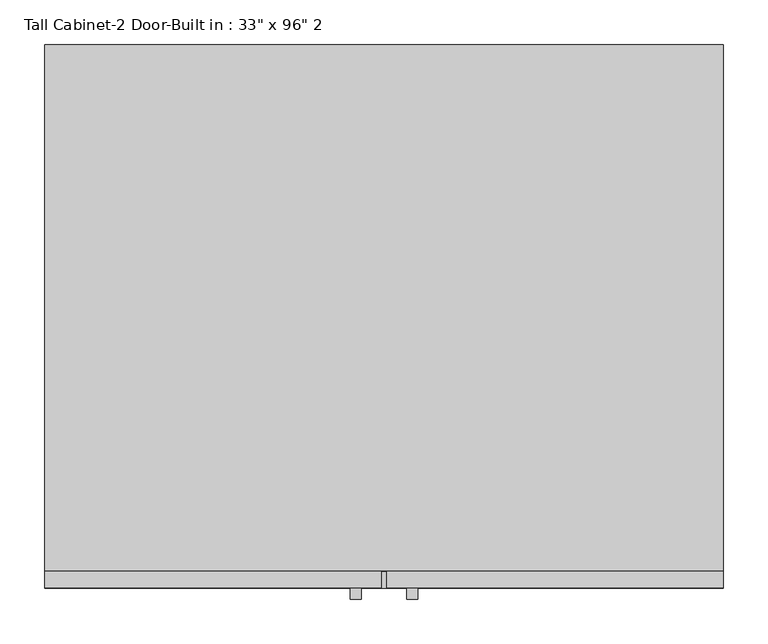
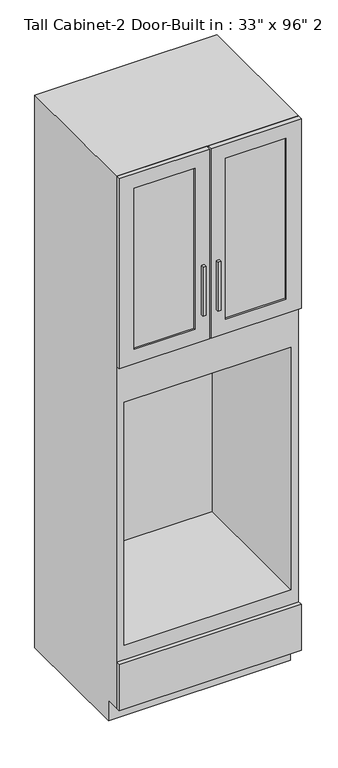
"""IFC4 building model written with IfcOpenShell, lengths in millimetres: furniture geometry."""

from ifc_helpers import new_model, si_unit, frame, origin, place, context, project, spatial, polyline, outline, extrude, faceted_brep, source, transform, mapped, element, save


def furniture_01bc0a7d(model_context):
    return source(origin(), model_context, "Body", "SolidModel", [
        faceted_brep([(399.7377049, -590.55, 90.4875), (399.7377049, -590.55, 2439.9875), (-362.2622951, -590.55, 2439.9875), (-362.2622951, -590.55, 90.4875), (-343.2122951, -590.55, 2420.9375), (380.6877049, -590.55, 2420.9375), (380.6877049, -590.55, 1601.7875), (-343.2122951, -590.55, 1601.7875), (367.9877049, -590.55, 357.1875), (-330.5122951, -590.55, 357.1875), (-330.5122951, -590.55, 1430.3375), (367.9877049, -590.55, 1430.3375), (-362.2622951, 0.0, 2439.9875), (399.7377049, 0.0, 2439.9875), (399.7377049, 0.0, 0.0), (-362.2622951, 0.0, 0.0), (399.7377049, -533.4, 90.4875), (399.7377049, -533.4, 0.0), (-362.2622951, -533.4, 0.0), (-362.2622951, -533.4, 90.4875), (380.6877049, -19.05, 2420.9375), (380.6877049, -19.05, 1601.7875), (-343.2122951, -19.05, 1601.7875), (-343.2122951, -19.05, 2420.9375), (367.9877049, -19.05, 357.1875), (-330.5122951, -19.05, 357.1875), (-330.5122951, -19.05, 1430.3375), (367.9877049, -19.05, 1430.3375)], [[[0, 1, 2, 3], [4, 5, 6, 7], [8, 9, 10, 11]], [[12, 13, 14, 15]], [[1, 0, 16, 17, 14, 13]], [[2, 1, 13, 12]], [[3, 2, 12, 15, 18, 19]], [[0, 3, 19, 16]], [[6, 5, 20, 21]], [[4, 7, 22, 23]], [[5, 4, 23, 20]], [[14, 17, 18, 15]], [[18, 17, 16, 19]], [[7, 6, 21, 22]], [[9, 8, 24, 25]], [[10, 9, 25, 26]], [[11, 10, 26, 27]], [[8, 11, 27, 24]], [[21, 20, 23, 22]], [[25, 24, 27, 26]]]),
        extrude(outline(polyline([(399.7377049, -609.6), (-362.2622951, -609.6), (-362.2622951, -590.55), (399.7377049, -590.55), (399.7377049, -609.6)])), frame((0.0, 0.0, 90.4875), z_axis=(0.0, 0.0, 1.0), x_axis=(1.0, 0.0, 0.0)), (0.0, 0.0, 1.0), 203.2),
        extrude(outline(polyline([(2439.9875, 15.5627049), (2439.9875, -362.2622951), (1601.7875, -362.2622951), (1601.7875, 15.5627049), (2439.9875, 15.5627049)]), holes=[polyline([(2376.4875, -44.7622951), (1665.2875, -44.7622951), (1665.2875, -298.7622951), (2376.4875, -298.7622951), (2376.4875, -44.7622951)])]), frame((0.0, -609.6, 0.0), z_axis=(0.0, 1.0, 0.0), x_axis=(0.0, 0.0, 1.0)), (0.0, 0.0, 1.0), 19.05),
        extrude(outline(polyline([(2439.9875, 21.9127049), (1601.7875, 21.9127049), (1601.7875, 399.7377049), (2439.9875, 399.7377049), (2439.9875, 21.9127049)]), holes=[polyline([(2376.4875, 336.2377049), (1665.2875, 336.2377049), (1665.2875, 82.2377049), (2376.4875, 82.2377049), (2376.4875, 336.2377049)])]), frame((0.0, -609.6, 0.0), z_axis=(0.0, 1.0, 0.0), x_axis=(0.0, 0.0, 1.0)), (0.0, 0.0, 1.0), 19.05),
        extrude(outline(polyline([(399.7377049, -609.6), (-362.2622951, -609.6), (-362.2622951, -590.55), (399.7377049, -590.55), (399.7377049, -609.6)])), frame((0.0, 0.0, 90.4875), z_axis=(0.0, 0.0, 1.0), x_axis=(1.0, 0.0, 0.0)), (0.0, 0.0, 1.0), 203.2),
        extrude(outline(polyline([(-6.6622951, -622.3), (-19.1945267, -622.3), (-19.1945267, -609.6), (-6.6622951, -609.6), (-6.6622951, -622.3)])), frame((0.0, 0.0, 1721.8417867), z_axis=(0.0, 0.0, 1.0), x_axis=(1.0, 0.0, 0.0)), (0.0, 0.0, 1.0), 215.9),
        extrude(outline(polyline([(56.6699365, -622.3), (44.1377049, -622.3), (44.1377049, -609.6), (56.6699365, -609.6), (56.6699365, -622.3)])), frame((0.0, 0.0, 1721.8417867), z_axis=(0.0, 0.0, 1.0), x_axis=(1.0, 0.0, 0.0)), (0.0, 0.0, 1.0), 215.9),
        extrude(outline(polyline([(-44.7622951, -603.25), (-298.7622951, -603.25), (-298.7622951, -596.9), (-44.7622951, -596.9), (-44.7622951, -603.25)])), frame((0.0, 0.0, 1665.2875), z_axis=(0.0, 0.0, 1.0), x_axis=(1.0, 0.0, 0.0)), (0.0, 0.0, 1.0), 711.2),
        extrude(outline(polyline([(336.2377049, -603.25), (82.2377049, -603.25), (82.2377049, -596.9), (336.2377049, -596.9), (336.2377049, -603.25)])), frame((0.0, 0.0, 1665.2875), z_axis=(0.0, 0.0, 1.0), x_axis=(1.0, 0.0, 0.0)), (0.0, 0.0, 1.0), 711.2),
    ])


if __name__ == "__main__":
    model = new_model("IFC4")
    model_context = context("Model", 3, world=origin())
    ifc_project = project(units=[si_unit("LENGTHUNIT", "METRE", prefix="MILLI")], contexts=[model_context])
    site = spatial("IfcSite", under=ifc_project)
    building = spatial("IfcBuilding", under=site)
    placement = place(None, origin())
    furniture_shape = furniture_01bc0a7d(model_context)
    element("IfcFurniture", 1, ObjectType="Tall Cabinet-2 Door-Built in : 33\" x 96\" 2", at=placement, inside=building, context=model_context, shape_type="MappedRepresentation", body=[
        mapped(furniture_shape, transform((0.0, 0.0, 0.0), x_axis=(1.0, 0.0, 0.0), y_axis=(0.0, 1.0, 0.0), z_axis=(0.0, 0.0, 1.0))),
    ])
    save(model, "model.ifc")

# Revit data of these elements
# Project information
#   Organization Name = "North Hills Home"
#   Building Name = "Barton Keep B&B"
#   Classification.Facility.Description = "Multiple Bedroom Family Residence"
#   Classification.Facility.Number = "11-16 11 17"
#   COBie.CreatedBy = "info@geappliances.com"
#   COBie.CreatedOn = "2017-07-20T03:49:28"
#   COBie.Facility.Name = "Barton Keep B&B"
#   COBie.Facility.Category = "11-16 11 17:Multiple Bedroom Family Residence"
#   COBie.Facility.ProjectName = "Barton Keep B&B"
#   COBie.Facility.LinearUnits = "Feet"
#   COBie.Facility.AreaUnits = "Square Feet"
#   COBie.Facility.VolumeUnits = "Cubic Feet"
#   COBie.Facility.CurrencyUnit = "Dollar"
#   COBie.Facility.AreaMeasurement = "Revit Default Area Calculation Method"
#   Project Issue Date = "2003-05-25"
#   Project Status = "Complete"
#   Client Name = "Eagale Noth America"
#   Project Address = "1002 East Swedesford Road King of Prussia, PA 19406 United States"
#   Project Name = "Barton Keep B&B"
#   Project Number = "Project Number"
# Type "Tall Cabinet-2 Door-Built in : 33\" x 96\" 2"
#   Assembly Code = "C1030410"
#   Type Comments = "21.5\"w 39.75\"h built-in"
#   Height = 8' - 0"
#   Depth = 2' - 0"
#   Height-Base of Built-in = 1' - 2"
#   Height-Built-in = 3' - 6 1/4"
#   Height-Upper Cabinet = 2' - 9"
#   Toe Depth = 0' - 3"
#   Toe Height = 0' - 3 1/2"
#   Width = 2' - 6"
#   COBie.Type = no
#   Cabinet Material = none
#   Door/Drawer Material = none
#   Handle Material = Cabinets - Handles
#   Panel Material = Glass
# Element 1 (IfcFurniture, "Tall Cabinet-2 Door-Built in : 33\" x 96\" 2")
#   Materials on its faces: "Cabinets", "Cabinets - Handles", "Glass"
# Materials
#   "Cabinets - Handles": class "Metal", colour RGB 57 57 57, transparency 0
#   "Glass": class "Glass", colour RGB 0 128 192, transparency 0.75, Description = "Soda Lime Glass", Cost = 0
#   "Cabinets": class "Miscellaneous", colour RGB 249 249 249, transparency 0
